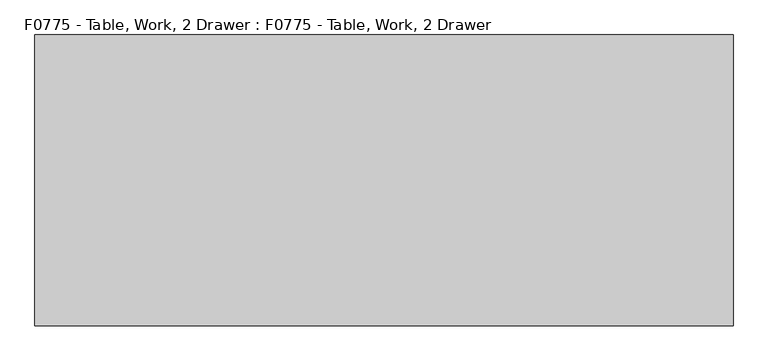
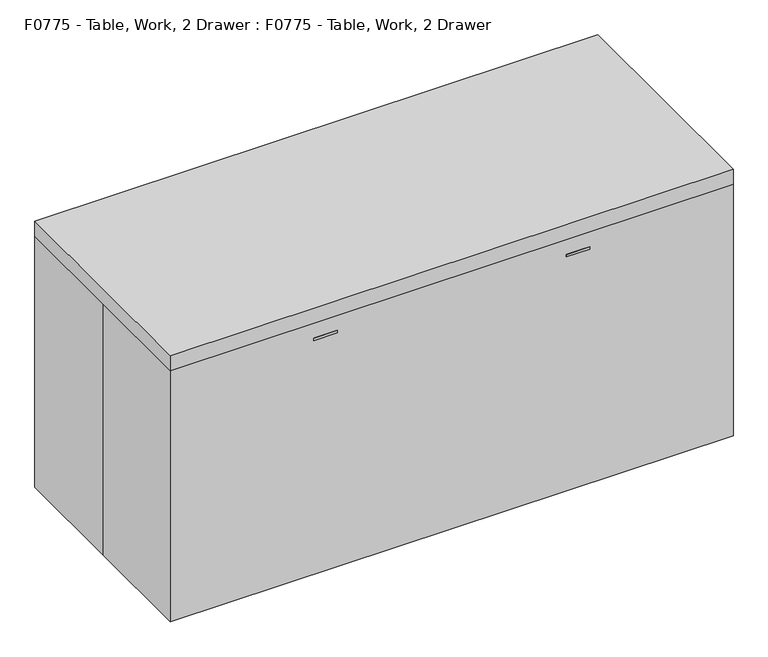
"""IFC4 building model written with IfcOpenShell, lengths in millimetres: proxy geometry, F0775 - Table, Work, 2 Drawer : F0775 - Table, Work, 2 Drawer."""

from ifc_helpers import new_model, si_unit, frame, origin, origin_with_axes, place, context, project, spatial, polyline, outline, extrude, source, transform, mapped, element, save


def f0775_table_work_2_drawer_f0775_table_work_2_drawer_e0e453b6(model_context):
    return source(origin(), model_context, "Body", "SweptSolid", [
        extrude(outline(polyline([(-447.8704593, -381.0), (-447.8704593, -365.05733), (-441.5204593, -365.05733), (-441.5204593, -377.75733), (-378.0204593, -377.75733), (-378.0204593, -365.05733), (-371.6704593, -365.05733), (-371.6704593, -381.0), (-447.8704593, -381.0)])), frame((0.0, 0.0, 803.5503382), z_axis=(0.0, 0.0, 1.0), x_axis=(1.0, 0.0, 0.0)), (0.0, 0.0, 1.0), 8.4842742),
        extrude(outline(polyline([(447.8704593, -381.0), (371.6704593, -381.0), (371.6704593, -365.05733), (378.0204593, -365.05733), (378.0204593, -377.75733), (441.5204593, -377.75733), (441.5204593, -365.05733), (447.8704593, -365.05733), (447.8704593, -381.0)])), frame((0.0, 0.0, 803.5503382), z_axis=(0.0, 0.0, 1.0), x_axis=(1.0, 0.0, 0.0)), (0.0, 0.0, 1.0), 8.4842742),
        extrude(outline(polyline([(-66.8704593, -365.05733), (-752.6704593, -365.05733), (-752.6704593, -355.6), (-66.8704593, -355.6), (-66.8704593, -365.05733)])), frame((0.0, 0.0, 762.0), z_axis=(0.0, 0.0, 1.0), x_axis=(1.0, 0.0, 0.0)), (0.0, 0.0, 1.0), 76.2),
        extrude(outline(polyline([(752.6704593, -365.05733), (66.8704593, -365.05733), (66.8704593, -355.6), (752.6704593, -355.6), (752.6704593, -365.05733)])), frame((0.0, 0.0, 762.0), z_axis=(0.0, 0.0, 1.0), x_axis=(1.0, 0.0, 0.0)), (0.0, 0.0, 1.0), 76.2),
        extrude(outline(polyline([(812.8, 355.6), (812.8, -355.6), (-812.8, -355.6), (-812.8, 355.6), (812.8, 355.6)])), frame((0.0, 0.0, 736.6), z_axis=(0.0, 0.0, 1.0), x_axis=(1.0, 0.0, 0.0)), (0.0, 0.0, 1.0), 127.0),
        extrude(outline(polyline([(914.4, 381.0), (914.4, -381.0), (-914.4, -381.0), (-914.4, 381.0), (914.4, 381.0)])), frame((0.0, 0.0, 863.6), z_axis=(0.0, 0.0, 1.0), x_axis=(1.0, 0.0, 0.0)), (0.0, 0.0, 1.0), 50.8),
        extrude(outline(polyline([(-812.8, 355.6), (-812.8, 279.4), (-889.0, 279.4), (-889.0, 355.6), (-812.8, 355.6)])), origin_with_axes(), (0.0, 0.0, 1.0), 863.6),
        extrude(outline(polyline([(812.8, 355.6), (889.0, 355.6), (889.0, 279.4), (812.8, 279.4), (812.8, 355.6)])), origin_with_axes(), (0.0, 0.0, 1.0), 863.6),
        extrude(outline(polyline([(-812.8, -355.6), (-889.0, -355.6), (-889.0, -279.4), (-812.8, -279.4), (-812.8, -355.6)])), origin_with_axes(), (0.0, 0.0, 1.0), 863.6),
        extrude(outline(polyline([(812.8, -355.6), (812.8, -279.4), (889.0, -279.4), (889.0, -355.6), (812.8, -355.6)])), origin_with_axes(), (0.0, 0.0, 1.0), 863.6),
        extrude(outline(polyline([(-914.4, 381.0), (914.4, 381.0), (914.4, -381.0), (-914.4, -381.0), (-914.4, 0.0), (-914.4, 381.0)])), origin_with_axes(), (0.0, 0.0, 1.0), 914.4),
    ])


if __name__ == "__main__":
    model = new_model("IFC4")
    model_context = context("Model", 3, world=origin())
    ifc_project = project(units=[si_unit("LENGTHUNIT", "METRE", prefix="MILLI")], contexts=[model_context])
    site = spatial("IfcSite", under=ifc_project)
    building = spatial("IfcBuilding", under=site)
    placement = place(None, origin())
    f0775_table_work_2_drawer_f0775_table_work_2_drawer_shape = f0775_table_work_2_drawer_f0775_table_work_2_drawer_e0e453b6(model_context)
    element("IfcBuildingElementProxy", 1, Name="F0775 - Table, Work, 2 Drawer : F0775 - Table, Work, 2 Drawer", ObjectType="F0775 - Table, Work, 2 Drawer : F0775 - Table, Work, 2 Drawer", at=placement, inside=building, context=model_context, shape_type="MappedRepresentation", body=[
        mapped(f0775_table_work_2_drawer_f0775_table_work_2_drawer_shape, transform((0.0, 0.0, 0.0), x_axis=(1.0, 0.0, 0.0), y_axis=(0.0, 1.0, 0.0), z_axis=(0.0, 0.0, 1.0))),
    ])
    save(model, "model.ifc")

# Revit data of these elements
# Type "F0775 - Table, Work, 2 Drawer : F0775 - Table, Work, 2 Drawer"
#   Watts2 = "0"
#   Watts1 = "0"
#   Unit_Issue = "EA"
#   UTIL_6_Misc = "-"
#   UTIL_5_NonMedGas = "-"
#   UTIL_4_MiscGas = "-"
#   UTIL_3_MedGas = "-"
#   UTIL_2_Elec = "-"
#   UTIL_1_WaterDrain = "-"
#   Nomenclature = "Table, Work, 2 Drawer"
#   NSN = "7110"
#   Location [instance default] = ""
#   JSN = "F0775"
#   Fund_Source_VA = "-"
#   Fund_Source_Navy = "-"
#   Fund_Source_Army = "-"
#   Fund_Source_AF = "-"
#   ELEC_Volts2 = "0"
#   ELEC_Volts1 = "0"
#   ELEC_Phase2 = "0"
#   ELEC_Phase1 = "0"
#   ELEC_HertzSwitch = "0"
#   ELEC_HertzDependent = "0"
#   ELEC_Hertz = "0"
#   ELEC_Amps2 = "0"
#   ELEC_Amps1 = "0"
#   DetailDescription = "Work table approximately 32\" high X 72\" wide X 30\" deep with two drawers and a hard wood top."
#   CAT_VA = "C"
#   CAT_Navy = "C"
#   CAT_IHS = "-"
#   CAT_Army = "C"
#   CAT_AF = "C"
#   BTUperhour = "0"
#   Weight_IP = 195
#   DIM_Width_IP = 6' - 0"
#   DIM_Height_IP = 3' - 0"
#   DIM_Depth_IP = 2' - 6"
# Element 1 (IfcBuildingElementProxy, "F0775 - Table, Work, 2 Drawer : F0775 - Table, Work, 2 Drawer")
#   Materials on its faces: "EquipSpace"
# Materials
#   "EquipSpace": class "Unassigned", colour RGB 221 217 195, transparency 0.5
